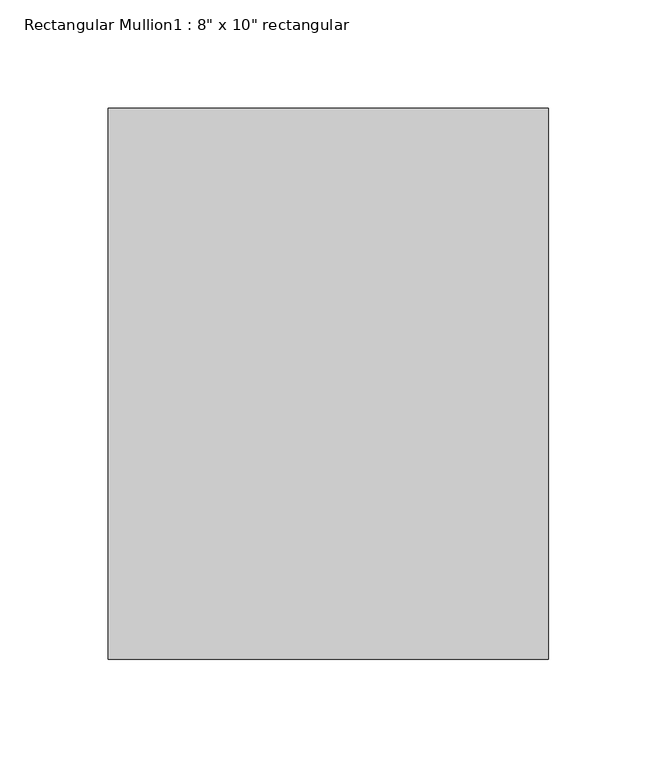
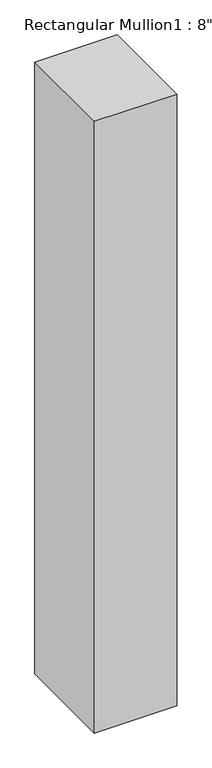
"""IFC4 building model written with IfcOpenShell, lengths in millimetres: member geometry."""

from ifc_helpers import new_model, si_unit, frame, origin, place, context, project, spatial, polyline, outline, extrude, source, transform, mapped, element, save


def member_ac1621ee(model_context):
    return source(origin(), model_context, "Body", "SweptSolid", [
        extrude(outline(polyline([(0.0, 127.0), (0.0, -127.0), (-203.2, -127.0), (-203.2, 127.0), (0.0, 127.0)])), frame((0.0, 0.0, -1593.8500097), z_axis=(0.0, 0.0, 1.0), x_axis=(1.0, 0.0, 0.0)), (0.0, 0.0, 1.0), 1593.8500097),
    ])


if __name__ == "__main__":
    model = new_model("IFC4")
    model_context = context("Model", 3, world=origin())
    ifc_project = project(units=[si_unit("LENGTHUNIT", "METRE", prefix="MILLI")], contexts=[model_context])
    site = spatial("IfcSite", under=ifc_project)
    building = spatial("IfcBuilding", under=site)
    placement = place(None, origin())
    member_shape = member_ac1621ee(model_context)
    element("IfcMember", 1, ObjectType="Rectangular Mullion1 : 8\" x 10\" rectangular", at=placement, inside=building, context=model_context, shape_type="MappedRepresentation", body=[
        mapped(member_shape, transform((0.0, 0.0, 0.0), x_axis=(1.0, 0.0, 0.0), y_axis=(0.0, 1.0, 0.0), z_axis=(0.0, 0.0, 1.0))),
    ])
    save(model, "model.ifc")

# Revit data of these elements
# Type "Rectangular Mullion1 : 8\" x 10\" rectangular"
#   built-in parameter 1007304 = 0.833333 (stored number, unit not read)
#   built-in parameter 1007301 = 0.333333 (stored number, unit not read)
#   built-in parameter 1007300 = 0.333333 (stored number, unit not read)
# Element 1 (IfcMember, "Rectangular Mullion1 : 8\" x 10\" rectangular")
#   Materials on its faces: "support-frame"
# Materials
#   "support-frame": class "Unassigned", colour RGB 233 233 233, transparency 0, Cost = 0
